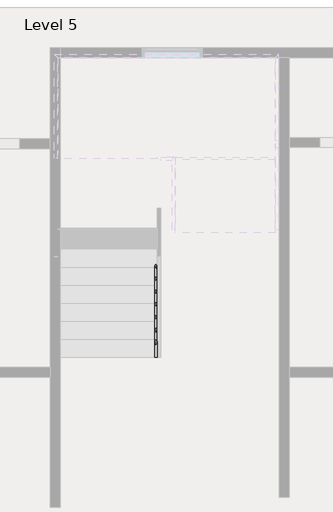
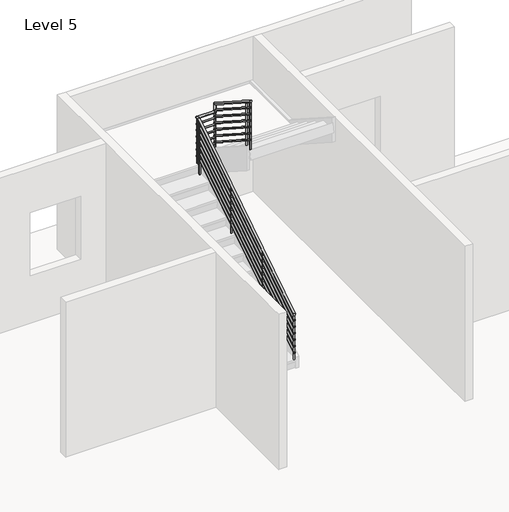
# One storey, part 6 of 7: 1 railing.
"""IFC4 building model written with IfcOpenShell, lengths in millimetres."""

from ifc_helpers import new_model, si_unit, point, frame, frame_2d, origin, place, context, project, spatial, circle_curve, ellipse_curve, trimmed, segment, composite_curve, outline, extrude, element, save
from ifc_brep_helpers import plane_surface, cylinder_surface, advanced_brep

model = new_model("IFC4")

# Units and contexts
model_context = context("Model", 3, world=origin())
ifc_project = project(units=[si_unit("LENGTHUNIT", "METRE", prefix="MILLI")], contexts=[model_context])

# Site, building, storey
site = spatial("IfcSite", under=ifc_project)
building = spatial("IfcBuilding", under=site)
storey = spatial("IfcBuildingStorey", under=building, Name="Level 5", Elevation=12500.0)

# Railing
placement = place(None, origin())
element("IfcRailing", 1, ObjectType="900mm Pipe", at=placement, inside=storey, context=model_context, shape_type="SolidModel", body=[
    advanced_brep(
    [(-504.8393676, 4284.7509075, 13552.7068065), (-544.8393676, 4284.7509075, 13552.7068065), (-504.8393676, 7315.616134, 15497.6470588), (-544.8393676, 7315.616134, 15497.6470588), (-504.8393676, 7337.8781803, 15497.6470588), (-544.8393676, 7377.8781803, 15497.6470588), (-201.3120949, 7337.8781803, 15497.6470588), (-201.3120949, 7377.8781803, 15497.6470588)],
    [
        (0, 1, ellipse_curve(frame((-524.8393676, 4284.7509075, 13552.7068065), z_axis=(0.0, -1.0, 0.0), x_axis=(0.0, 0.0, -1.0)), 23.7637817, 20.0)),
        (1, 0, ellipse_curve(frame((-524.8393676, 4284.7509075, 13552.7068065), z_axis=(0.0, -1.0, 0.0), x_axis=(0.0, 0.0, -1.0)), 23.7637817, 20.0)),
        (0, 2),
        (2, 3, ellipse_curve(frame((-524.8393676, 7315.616134, 15497.6470588), z_axis=(0.0, -0.9595876426002529, -0.28140994326585084), x_axis=(0.0, 0.2814099432658509, -0.959587642600253)), 20.8422859, 20.0)),
        (3, 1),
        (3, 2, ellipse_curve(frame((-524.8393676, 7315.616134, 15497.6470588), z_axis=(0.0, -0.9595876426002529, -0.28140994326585084), x_axis=(0.0, 0.2814099432658509, -0.959587642600253)), 20.8422859, 20.0)),
        (2, 4),
        (4, 5, ellipse_curve(frame((-524.8393676, 7357.8781803, 15497.6470588), z_axis=(-0.7071067811865475, -0.7071067811865475, 0.0), x_axis=(0.7071067811865474, -0.7071067811865476, 0.0)), 28.2842712, 20.0)),
        (5, 3),
        (5, 4, ellipse_curve(frame((-524.8393676, 7357.8781803, 15497.6470588), z_axis=(-0.7071067811865475, -0.7071067811865475, 0.0), x_axis=(0.7071067811865474, -0.7071067811865476, 0.0)), 28.2842712, 20.0)),
        (6, 7, ellipse_curve(frame((-201.3120949, 7357.8781803, 15497.6470588), z_axis=(0.7071067811865476, 0.0, 0.7071067811865476), x_axis=(-0.7071067811865474, 0.0, 0.7071067811865476)), 28.2842712, 20.0)),
        (7, 6, ellipse_curve(frame((-201.3120949, 7357.8781803, 15497.6470588), z_axis=(0.7071067811865476, 0.0, 0.7071067811865476), x_axis=(-0.7071067811865474, 0.0, 0.7071067811865476)), 28.2842712, 20.0)),
        (4, 6),
        (7, 5),
    ],
    [
        plane_surface(frame((-524.8393676, 4284.7509075, 13576.4705882), z_axis=(0.0, -1.0, 0.0), x_axis=(0.0, 0.0, 1.0))),
        cylinder_surface(frame((-524.8393676, 4295.5524077, 13559.6382505), z_axis=(0.0, -0.8416168876622212, -0.5400750081254975), x_axis=(-1.0, 0.0, 0.0)), 20.0),
        cylinder_surface(frame((-524.8393676, 7309.7509075, 15497.6470588), z_axis=(0.0, -1.0, 0.0), x_axis=(-1.0, 0.0, 0.0)), 20.0),
        plane_surface(frame((-221.3120949, 7357.8781803, 15517.6470588), z_axis=(0.7071067811865476, 0.0, 0.7071067811865476), x_axis=(0.7071067811865476, 0.0, -0.7071067811865476))),
        cylinder_surface(frame((-524.8393676, 7357.8781803, 15497.6470588), z_axis=(-1.0, 0.0, 0.0), x_axis=(0.0, 1.0, 0.0)), 20.0),
    ],
    [
        (0, [[1, 2]]),
        (1, [[-1, 3, 4, 5]]),
        (1, [[-2, -5, 6, -3]]),
        (2, [[-4, 7, 8, 9]]),
        (2, [[-6, -9, 10, -7]]),
        (3, [[11, 12]]),
        (4, [[-8, 13, -12, 14]]),
        (4, [[-10, -14, -11, -13]]),
    ],
),
    advanced_brep(
    [(-201.3120949, 7337.8781803, 15497.6470588), (-201.3120949, 7377.8781803, 15497.6470588), (-201.3120949, 7337.8781803, 15643.124843), (-201.3120949, 7377.8781803, 15664.9839572)],
    [
        (0, 1, ellipse_curve(frame((-201.3120949, 7357.8781803, 15497.6470588), z_axis=(-0.7071067811865476, 0.0, -0.7071067811865476), x_axis=(0.7071067811865476, 0.0, -0.7071067811865474)), 28.2842712, 20.0)),
        (1, 0, ellipse_curve(frame((-201.3120949, 7357.8781803, 15497.6470588), z_axis=(-0.7071067811865476, 0.0, -0.7071067811865476), x_axis=(0.7071067811865476, 0.0, -0.7071067811865474)), 28.2842712, 20.0)),
        (2, 3, ellipse_curve(frame((-201.3120949, 7357.8781803, 15654.0544001), z_axis=(0.0, -0.47954405004884676, 0.877517808402057), x_axis=(0.0, -0.8775178084020571, -0.47954405004884676)), 22.7915602, 20.0)),
        (3, 2, ellipse_curve(frame((-201.3120949, 7357.8781803, 15654.0544001), z_axis=(0.0, -0.47954405004884676, 0.877517808402057), x_axis=(0.0, -0.8775178084020571, -0.47954405004884676)), 22.7915602, 20.0)),
        (0, 2),
        (3, 1),
    ],
    [
        plane_surface(frame((-201.3120949, 7357.8781803, 15497.6470588), z_axis=(-0.7071067811865476, 0.0, -0.7071067811865476), x_axis=(0.7071067811865476, 0.0, -0.7071067811865476))),
        plane_surface(frame((-201.3120949, 7357.8781803, 15654.0544001), z_axis=(0.0, -0.47954405004884676, 0.877517808402057), x_axis=(1.0, 0.0, 0.0))),
        cylinder_surface(frame((-201.3120949, 7357.8781803, 15497.6470588), z_axis=(0.0, 0.0, -1.0), x_axis=(0.0, 1.0, 0.0)), 20.0),
    ],
    [
        (0, [[1, 2]]),
        (1, [[3, 4]]),
        (2, [[-1, 5, -4, 6]]),
        (2, [[-2, -6, -3, -5]]),
    ],
),
    advanced_brep(
    [(-221.3120949, 7357.8781803, 15654.0544001), (-181.3120949, 7357.8781803, 15654.0544001), (-221.3120949, 6232.4781803, 16376.2362183), (-181.3120949, 6232.4781803, 16376.2362183)],
    [
        (0, 1, ellipse_curve(frame((-201.3120949, 7357.8781803, 15654.0544001), z_axis=(0.0, 0.47954405004884676, -0.877517808402057), x_axis=(0.0, 0.8775178084020568, 0.47954405004884676)), 22.7915602, 20.0)),
        (1, 0, ellipse_curve(frame((-201.3120949, 7357.8781803, 15654.0544001), z_axis=(0.0, 0.47954405004884676, -0.877517808402057), x_axis=(0.0, 0.8775178084020568, 0.47954405004884676)), 22.7915602, 20.0)),
        (2, 3, ellipse_curve(frame((-201.3120949, 6232.4781803, 16376.2362183), z_axis=(0.0, -1.0, 0.0), x_axis=(0.0, 0.0, -1.0)), 23.7637817, 20.0)),
        (3, 2, ellipse_curve(frame((-201.3120949, 6232.4781803, 16376.2362183), z_axis=(0.0, -1.0, 0.0), x_axis=(0.0, 0.0, -1.0)), 23.7637817, 20.0)),
        (0, 2),
        (3, 1),
    ],
    [
        plane_surface(frame((-201.3120949, 7377.8781803, 15664.9839572), z_axis=(0.0, 0.47954405004884676, -0.877517808402057), x_axis=(1.0, 0.0, 0.0))),
        plane_surface(frame((-201.3120949, 6232.4781803, 16400.0), z_axis=(0.0, -1.0, 0.0), x_axis=(0.0, 0.0, -1.0))),
        cylinder_surface(frame((-201.3120949, 7367.0766801, 15648.1516195), z_axis=(0.0, 0.8416168876622208, -0.5400750081254984), x_axis=(1.0, 0.0, 0.0)), 20.0),
    ],
    [
        (0, [[1, 2]]),
        (1, [[3, 4]]),
        (2, [[-1, 5, -4, 6]]),
        (2, [[-2, -6, -3, -5]]),
    ],
),
    advanced_brep(
    [(-539.8393676, 4284.7509075, 13433.647752), (-509.8393676, 4284.7509075, 13433.647752), (-539.8393676, 7309.7509075, 15374.8242225), (-509.8393676, 7309.7509075, 15374.8242225)],
    [
        (0, 1, ellipse_curve(frame((-524.8393676, 4284.7509075, 13433.647752), z_axis=(0.0, -1.0, 0.0), x_axis=(0.0, 0.0, -1.0)), 17.8228363, 15.0)),
        (1, 0, ellipse_curve(frame((-524.8393676, 4284.7509075, 13433.647752), z_axis=(0.0, -1.0, 0.0), x_axis=(0.0, 0.0, -1.0)), 17.8228363, 15.0)),
        (2, 3, ellipse_curve(frame((-524.8393676, 7309.7509075, 15374.8242225), z_axis=(0.0, 1.0, 0.0), x_axis=(0.0, 0.0, -1.0)), 17.8228363, 15.0)),
        (3, 2, ellipse_curve(frame((-524.8393676, 7309.7509075, 15374.8242225), z_axis=(0.0, 1.0, 0.0), x_axis=(0.0, 0.0, -1.0)), 17.8228363, 15.0)),
        (0, 2),
        (3, 1),
    ],
    [
        plane_surface(frame((-524.8393676, 4284.7509075, 13451.4705882), z_axis=(0.0, -1.0, 0.0), x_axis=(0.0, 0.0, 1.0))),
        plane_surface(frame((-524.8393676, 7309.7509075, 15392.6470588), z_axis=(0.0, 1.0, 0.0), x_axis=(0.0, 0.0, 1.0))),
        cylinder_surface(frame((-524.8393676, 4292.8520327, 13438.8463349), z_axis=(0.0, -0.8416168876622212, -0.5400750081254975), x_axis=(1.0, 0.0, 0.0)), 15.0),
    ],
    [
        (0, [[1, 2]]),
        (1, [[3, 4]]),
        (2, [[-1, 5, -4, 6]]),
        (2, [[-2, -6, -3, -5]]),
    ],
),
    advanced_brep(
    [(-539.8393676, 7309.7509075, 15377.6470588), (-509.8393676, 7309.7509075, 15377.6470588), (-539.8393676, 7342.8781803, 15377.6470588), (-509.8393676, 7342.8781803, 15377.6470588)],
    [
        (0, 1, circle_curve(frame((-524.8393676, 7309.7509075, 15377.6470588), z_axis=(0.0, -1.0, 0.0), x_axis=(1.0, 0.0, 0.0)), 15.0)),
        (1, 0, circle_curve(frame((-524.8393676, 7309.7509075, 15377.6470588), z_axis=(0.0, -1.0, 0.0), x_axis=(1.0, 0.0, 0.0)), 15.0)),
        (2, 3, circle_curve(frame((-524.8393676, 7342.8781803, 15377.6470588), z_axis=(0.0, 1.0, 0.0), x_axis=(1.0, 0.0, 0.0)), 15.0)),
        (3, 2, circle_curve(frame((-524.8393676, 7342.8781803, 15377.6470588), z_axis=(0.0, 1.0, 0.0), x_axis=(1.0, 0.0, 0.0)), 15.0)),
        (0, 2),
        (3, 1),
    ],
    [
        plane_surface(frame((-524.8393676, 7309.7509075, 15392.6470588), z_axis=(0.0, -1.0, 0.0), x_axis=(0.0, 0.0, 1.0))),
        plane_surface(frame((-524.8393676, 7342.8781803, 15392.6470588), z_axis=(0.0, 1.0, 0.0), x_axis=(0.0, 0.0, 1.0))),
        cylinder_surface(frame((-524.8393676, 7309.7509075, 15377.6470588), z_axis=(0.0, -1.0, 0.0), x_axis=(1.0, 0.0, 0.0)), 15.0),
    ],
    [
        (0, [[1, 2]]),
        (1, [[3, 4]]),
        (2, [[-1, 5, -4, 6]]),
        (2, [[-2, -6, -3, -5]]),
    ],
),
    advanced_brep(
    [(-539.8393676, 7372.8781803, 15377.6470588), (-539.8393676, 7342.8781803, 15377.6470588), (-216.3120949, 7372.8781803, 15377.6470588), (-216.3120949, 7342.8781803, 15377.6470588)],
    [
        (0, 1, circle_curve(frame((-539.8393676, 7357.8781803, 15377.6470588), z_axis=(-1.0, 0.0, 0.0), x_axis=(0.0, -1.0, 0.0)), 15.0)),
        (1, 0, circle_curve(frame((-539.8393676, 7357.8781803, 15377.6470588), z_axis=(-1.0, 0.0, 0.0), x_axis=(0.0, -1.0, 0.0)), 15.0)),
        (2, 3, circle_curve(frame((-216.3120949, 7357.8781803, 15377.6470588), z_axis=(1.0, 0.0, 0.0), x_axis=(0.0, -1.0, 0.0)), 15.0)),
        (3, 2, circle_curve(frame((-216.3120949, 7357.8781803, 15377.6470588), z_axis=(1.0, 0.0, 0.0), x_axis=(0.0, -1.0, 0.0)), 15.0)),
        (0, 2),
        (3, 1),
    ],
    [
        plane_surface(frame((-539.8393676, 7357.8781803, 15392.6470588), z_axis=(-1.0, 0.0, 0.0), x_axis=(0.0, 1.0, 0.0))),
        plane_surface(frame((-216.3120949, 7357.8781803, 15392.6470588), z_axis=(1.0, 0.0, 0.0), x_axis=(0.0, 1.0, 0.0))),
        cylinder_surface(frame((-539.8393676, 7357.8781803, 15377.6470588), z_axis=(-1.0, 0.0, 0.0), x_axis=(0.0, -1.0, 0.0)), 15.0),
    ],
    [
        (0, [[1, 2]]),
        (1, [[3, 4]]),
        (2, [[-1, 5, -4, 6]]),
        (2, [[-2, -6, -3, -5]]),
    ],
),
    advanced_brep(
    [(-186.3120949, 7372.8781803, 15525.3696771), (-216.3120949, 7372.8781803, 15525.3696771), (-186.3120949, 6232.4781803, 16257.1771637), (-216.3120949, 6232.4781803, 16257.1771637)],
    [
        (0, 1, ellipse_curve(frame((-201.3120949, 7372.8781803, 15525.3696771), z_axis=(0.0, 1.0, 0.0), x_axis=(0.0, 0.0, -1.0)), 17.8228363, 15.0)),
        (1, 0, ellipse_curve(frame((-201.3120949, 7372.8781803, 15525.3696771), z_axis=(0.0, 1.0, 0.0), x_axis=(0.0, 0.0, -1.0)), 17.8228363, 15.0)),
        (2, 3, ellipse_curve(frame((-201.3120949, 6232.4781803, 16257.1771637), z_axis=(0.0, -1.0, 0.0), x_axis=(0.0, 0.0, -1.0)), 17.8228363, 15.0)),
        (3, 2, ellipse_curve(frame((-201.3120949, 6232.4781803, 16257.1771637), z_axis=(0.0, -1.0, 0.0), x_axis=(0.0, 0.0, -1.0)), 17.8228363, 15.0)),
        (0, 2),
        (3, 1),
    ],
    [
        plane_surface(frame((-201.3120949, 7372.8781803, 15543.1925134), z_axis=(0.0, 1.0, 0.0), x_axis=(0.0, 0.0, -1.0))),
        plane_surface(frame((-201.3120949, 6232.4781803, 16275.0), z_axis=(0.0, -1.0, 0.0), x_axis=(0.0, 0.0, -1.0))),
        cylinder_surface(frame((-201.3120949, 7364.7770552, 15530.5682601), z_axis=(0.0, 0.8416168876622208, -0.5400750081254984), x_axis=(-1.0, 0.0, 0.0)), 15.0),
    ],
    [
        (0, [[1, 2]]),
        (1, [[3, 4]]),
        (2, [[-1, 5, -4, 6]]),
        (2, [[-2, -6, -3, -5]]),
    ],
),
    advanced_brep(
    [(-539.8393676, 4284.7509075, 13308.647752), (-509.8393676, 4284.7509075, 13308.647752), (-539.8393676, 7309.7509075, 15249.8242225), (-509.8393676, 7309.7509075, 15249.8242225)],
    [
        (0, 1, ellipse_curve(frame((-524.8393676, 4284.7509075, 13308.647752), z_axis=(0.0, -1.0, 0.0), x_axis=(0.0, 0.0, -1.0)), 17.8228363, 15.0)),
        (1, 0, ellipse_curve(frame((-524.8393676, 4284.7509075, 13308.647752), z_axis=(0.0, -1.0, 0.0), x_axis=(0.0, 0.0, -1.0)), 17.8228363, 15.0)),
        (2, 3, ellipse_curve(frame((-524.8393676, 7309.7509075, 15249.8242225), z_axis=(0.0, 1.0, 0.0), x_axis=(0.0, 0.0, -1.0)), 17.8228363, 15.0)),
        (3, 2, ellipse_curve(frame((-524.8393676, 7309.7509075, 15249.8242225), z_axis=(0.0, 1.0, 0.0), x_axis=(0.0, 0.0, -1.0)), 17.8228363, 15.0)),
        (0, 2),
        (3, 1),
    ],
    [
        plane_surface(frame((-524.8393676, 4284.7509075, 13326.4705882), z_axis=(0.0, -1.0, 0.0), x_axis=(0.0, 0.0, 1.0))),
        plane_surface(frame((-524.8393676, 7309.7509075, 15267.6470588), z_axis=(0.0, 1.0, 0.0), x_axis=(0.0, 0.0, 1.0))),
        cylinder_surface(frame((-524.8393676, 4292.8520327, 13313.8463349), z_axis=(0.0, -0.8416168876622212, -0.5400750081254975), x_axis=(1.0, 0.0, 0.0)), 15.0),
    ],
    [
        (0, [[1, 2]]),
        (1, [[3, 4]]),
        (2, [[-1, 5, -4, 6]]),
        (2, [[-2, -6, -3, -5]]),
    ],
),
    advanced_brep(
    [(-539.8393676, 7309.7509075, 15252.6470588), (-509.8393676, 7309.7509075, 15252.6470588), (-539.8393676, 7342.8781803, 15252.6470588), (-509.8393676, 7342.8781803, 15252.6470588)],
    [
        (0, 1, circle_curve(frame((-524.8393676, 7309.7509075, 15252.6470588), z_axis=(0.0, -1.0, 0.0), x_axis=(1.0, 0.0, 0.0)), 15.0)),
        (1, 0, circle_curve(frame((-524.8393676, 7309.7509075, 15252.6470588), z_axis=(0.0, -1.0, 0.0), x_axis=(1.0, 0.0, 0.0)), 15.0)),
        (2, 3, circle_curve(frame((-524.8393676, 7342.8781803, 15252.6470588), z_axis=(0.0, 1.0, 0.0), x_axis=(1.0, 0.0, 0.0)), 15.0)),
        (3, 2, circle_curve(frame((-524.8393676, 7342.8781803, 15252.6470588), z_axis=(0.0, 1.0, 0.0), x_axis=(1.0, 0.0, 0.0)), 15.0)),
        (0, 2),
        (3, 1),
    ],
    [
        plane_surface(frame((-524.8393676, 7309.7509075, 15267.6470588), z_axis=(0.0, -1.0, 0.0), x_axis=(0.0, 0.0, 1.0))),
        plane_surface(frame((-524.8393676, 7342.8781803, 15267.6470588), z_axis=(0.0, 1.0, 0.0), x_axis=(0.0, 0.0, 1.0))),
        cylinder_surface(frame((-524.8393676, 7309.7509075, 15252.6470588), z_axis=(0.0, -1.0, 0.0), x_axis=(1.0, 0.0, 0.0)), 15.0),
    ],
    [
        (0, [[1, 2]]),
        (1, [[3, 4]]),
        (2, [[-1, 5, -4, 6]]),
        (2, [[-2, -6, -3, -5]]),
    ],
),
    advanced_brep(
    [(-539.8393676, 7372.8781803, 15252.6470588), (-539.8393676, 7342.8781803, 15252.6470588), (-216.3120949, 7372.8781803, 15252.6470588), (-216.3120949, 7342.8781803, 15252.6470588)],
    [
        (0, 1, circle_curve(frame((-539.8393676, 7357.8781803, 15252.6470588), z_axis=(-1.0, 0.0, 0.0), x_axis=(0.0, -1.0, 0.0)), 15.0)),
        (1, 0, circle_curve(frame((-539.8393676, 7357.8781803, 15252.6470588), z_axis=(-1.0, 0.0, 0.0), x_axis=(0.0, -1.0, 0.0)), 15.0)),
        (2, 3, circle_curve(frame((-216.3120949, 7357.8781803, 15252.6470588), z_axis=(1.0, 0.0, 0.0), x_axis=(0.0, -1.0, 0.0)), 15.0)),
        (3, 2, circle_curve(frame((-216.3120949, 7357.8781803, 15252.6470588), z_axis=(1.0, 0.0, 0.0), x_axis=(0.0, -1.0, 0.0)), 15.0)),
        (0, 2),
        (3, 1),
    ],
    [
        plane_surface(frame((-539.8393676, 7357.8781803, 15267.6470588), z_axis=(-1.0, 0.0, 0.0), x_axis=(0.0, 1.0, 0.0))),
        plane_surface(frame((-216.3120949, 7357.8781803, 15267.6470588), z_axis=(1.0, 0.0, 0.0), x_axis=(0.0, 1.0, 0.0))),
        cylinder_surface(frame((-539.8393676, 7357.8781803, 15252.6470588), z_axis=(-1.0, 0.0, 0.0), x_axis=(0.0, -1.0, 0.0)), 15.0),
    ],
    [
        (0, [[1, 2]]),
        (1, [[3, 4]]),
        (2, [[-1, 5, -4, 6]]),
        (2, [[-2, -6, -3, -5]]),
    ],
),
    advanced_brep(
    [(-186.3120949, 7372.8781803, 15400.3696771), (-216.3120949, 7372.8781803, 15400.3696771), (-186.3120949, 6232.4781803, 16132.1771637), (-216.3120949, 6232.4781803, 16132.1771637)],
    [
        (0, 1, ellipse_curve(frame((-201.3120949, 7372.8781803, 15400.3696771), z_axis=(0.0, 1.0, 0.0), x_axis=(0.0, 0.0, -1.0)), 17.8228363, 15.0)),
        (1, 0, ellipse_curve(frame((-201.3120949, 7372.8781803, 15400.3696771), z_axis=(0.0, 1.0, 0.0), x_axis=(0.0, 0.0, -1.0)), 17.8228363, 15.0)),
        (2, 3, ellipse_curve(frame((-201.3120949, 6232.4781803, 16132.1771637), z_axis=(0.0, -1.0, 0.0), x_axis=(0.0, 0.0, -1.0)), 17.8228363, 15.0)),
        (3, 2, ellipse_curve(frame((-201.3120949, 6232.4781803, 16132.1771637), z_axis=(0.0, -1.0, 0.0), x_axis=(0.0, 0.0, -1.0)), 17.8228363, 15.0)),
        (0, 2),
        (3, 1),
    ],
    [
        plane_surface(frame((-201.3120949, 7372.8781803, 15418.1925134), z_axis=(0.0, 1.0, 0.0), x_axis=(0.0, 0.0, -1.0))),
        plane_surface(frame((-201.3120949, 6232.4781803, 16150.0), z_axis=(0.0, -1.0, 0.0), x_axis=(0.0, 0.0, -1.0))),
        cylinder_surface(frame((-201.3120949, 7364.7770552, 15405.5682601), z_axis=(0.0, 0.8416168876622208, -0.5400750081254984), x_axis=(-1.0, 0.0, 0.0)), 15.0),
    ],
    [
        (0, [[1, 2]]),
        (1, [[3, 4]]),
        (2, [[-1, 5, -4, 6]]),
        (2, [[-2, -6, -3, -5]]),
    ],
),
    advanced_brep(
    [(-539.8393676, 4284.7509075, 13183.647752), (-509.8393676, 4284.7509075, 13183.647752), (-539.8393676, 7309.7509075, 15124.8242225), (-509.8393676, 7309.7509075, 15124.8242225)],
    [
        (0, 1, ellipse_curve(frame((-524.8393676, 4284.7509075, 13183.647752), z_axis=(0.0, -1.0, 0.0), x_axis=(0.0, 0.0, -1.0)), 17.8228363, 15.0)),
        (1, 0, ellipse_curve(frame((-524.8393676, 4284.7509075, 13183.647752), z_axis=(0.0, -1.0, 0.0), x_axis=(0.0, 0.0, -1.0)), 17.8228363, 15.0)),
        (2, 3, ellipse_curve(frame((-524.8393676, 7309.7509075, 15124.8242225), z_axis=(0.0, 1.0, 0.0), x_axis=(0.0, 0.0, -1.0)), 17.8228363, 15.0)),
        (3, 2, ellipse_curve(frame((-524.8393676, 7309.7509075, 15124.8242225), z_axis=(0.0, 1.0, 0.0), x_axis=(0.0, 0.0, -1.0)), 17.8228363, 15.0)),
        (0, 2),
        (3, 1),
    ],
    [
        plane_surface(frame((-524.8393676, 4284.7509075, 13201.4705882), z_axis=(0.0, -1.0, 0.0), x_axis=(0.0, 0.0, 1.0))),
        plane_surface(frame((-524.8393676, 7309.7509075, 15142.6470588), z_axis=(0.0, 1.0, 0.0), x_axis=(0.0, 0.0, 1.0))),
        cylinder_surface(frame((-524.8393676, 4292.8520327, 13188.8463349), z_axis=(0.0, -0.8416168876622212, -0.5400750081254975), x_axis=(1.0, 0.0, 0.0)), 15.0),
    ],
    [
        (0, [[1, 2]]),
        (1, [[3, 4]]),
        (2, [[-1, 5, -4, 6]]),
        (2, [[-2, -6, -3, -5]]),
    ],
),
    advanced_brep(
    [(-539.8393676, 7309.7509075, 15127.6470588), (-509.8393676, 7309.7509075, 15127.6470588), (-539.8393676, 7342.8781803, 15127.6470588), (-509.8393676, 7342.8781803, 15127.6470588)],
    [
        (0, 1, circle_curve(frame((-524.8393676, 7309.7509075, 15127.6470588), z_axis=(0.0, -1.0, 0.0), x_axis=(1.0, 0.0, 0.0)), 15.0)),
        (1, 0, circle_curve(frame((-524.8393676, 7309.7509075, 15127.6470588), z_axis=(0.0, -1.0, 0.0), x_axis=(1.0, 0.0, 0.0)), 15.0)),
        (2, 3, circle_curve(frame((-524.8393676, 7342.8781803, 15127.6470588), z_axis=(0.0, 1.0, 0.0), x_axis=(1.0, 0.0, 0.0)), 15.0)),
        (3, 2, circle_curve(frame((-524.8393676, 7342.8781803, 15127.6470588), z_axis=(0.0, 1.0, 0.0), x_axis=(1.0, 0.0, 0.0)), 15.0)),
        (0, 2),
        (3, 1),
    ],
    [
        plane_surface(frame((-524.8393676, 7309.7509075, 15142.6470588), z_axis=(0.0, -1.0, 0.0), x_axis=(0.0, 0.0, 1.0))),
        plane_surface(frame((-524.8393676, 7342.8781803, 15142.6470588), z_axis=(0.0, 1.0, 0.0), x_axis=(0.0, 0.0, 1.0))),
        cylinder_surface(frame((-524.8393676, 7309.7509075, 15127.6470588), z_axis=(0.0, -1.0, 0.0), x_axis=(1.0, 0.0, 0.0)), 15.0),
    ],
    [
        (0, [[1, 2]]),
        (1, [[3, 4]]),
        (2, [[-1, 5, -4, 6]]),
        (2, [[-2, -6, -3, -5]]),
    ],
),
    advanced_brep(
    [(-539.8393676, 7372.8781803, 15127.6470588), (-539.8393676, 7342.8781803, 15127.6470588), (-216.3120949, 7372.8781803, 15127.6470588), (-216.3120949, 7342.8781803, 15127.6470588)],
    [
        (0, 1, circle_curve(frame((-539.8393676, 7357.8781803, 15127.6470588), z_axis=(-1.0, 0.0, 0.0), x_axis=(0.0, -1.0, 0.0)), 15.0)),
        (1, 0, circle_curve(frame((-539.8393676, 7357.8781803, 15127.6470588), z_axis=(-1.0, 0.0, 0.0), x_axis=(0.0, -1.0, 0.0)), 15.0)),
        (2, 3, circle_curve(frame((-216.3120949, 7357.8781803, 15127.6470588), z_axis=(1.0, 0.0, 0.0), x_axis=(0.0, -1.0, 0.0)), 15.0)),
        (3, 2, circle_curve(frame((-216.3120949, 7357.8781803, 15127.6470588), z_axis=(1.0, 0.0, 0.0), x_axis=(0.0, -1.0, 0.0)), 15.0)),
        (0, 2),
        (3, 1),
    ],
    [
        plane_surface(frame((-539.8393676, 7357.8781803, 15142.6470588), z_axis=(-1.0, 0.0, 0.0), x_axis=(0.0, 1.0, 0.0))),
        plane_surface(frame((-216.3120949, 7357.8781803, 15142.6470588), z_axis=(1.0, 0.0, 0.0), x_axis=(0.0, 1.0, 0.0))),
        cylinder_surface(frame((-539.8393676, 7357.8781803, 15127.6470588), z_axis=(-1.0, 0.0, 0.0), x_axis=(0.0, -1.0, 0.0)), 15.0),
    ],
    [
        (0, [[1, 2]]),
        (1, [[3, 4]]),
        (2, [[-1, 5, -4, 6]]),
        (2, [[-2, -6, -3, -5]]),
    ],
),
    advanced_brep(
    [(-186.3120949, 7372.8781803, 15275.3696771), (-216.3120949, 7372.8781803, 15275.3696771), (-186.3120949, 6232.4781803, 16007.1771637), (-216.3120949, 6232.4781803, 16007.1771637)],
    [
        (0, 1, ellipse_curve(frame((-201.3120949, 7372.8781803, 15275.3696771), z_axis=(0.0, 1.0, 0.0), x_axis=(0.0, 0.0, -1.0)), 17.8228363, 15.0)),
        (1, 0, ellipse_curve(frame((-201.3120949, 7372.8781803, 15275.3696771), z_axis=(0.0, 1.0, 0.0), x_axis=(0.0, 0.0, -1.0)), 17.8228363, 15.0)),
        (2, 3, ellipse_curve(frame((-201.3120949, 6232.4781803, 16007.1771637), z_axis=(0.0, -1.0, 0.0), x_axis=(0.0, 0.0, -1.0)), 17.8228363, 15.0)),
        (3, 2, ellipse_curve(frame((-201.3120949, 6232.4781803, 16007.1771637), z_axis=(0.0, -1.0, 0.0), x_axis=(0.0, 0.0, -1.0)), 17.8228363, 15.0)),
        (0, 2),
        (3, 1),
    ],
    [
        plane_surface(frame((-201.3120949, 7372.8781803, 15293.1925134), z_axis=(0.0, 1.0, 0.0), x_axis=(0.0, 0.0, -1.0))),
        plane_surface(frame((-201.3120949, 6232.4781803, 16025.0), z_axis=(0.0, -1.0, 0.0), x_axis=(0.0, 0.0, -1.0))),
        cylinder_surface(frame((-201.3120949, 7364.7770552, 15280.5682601), z_axis=(0.0, 0.8416168876622208, -0.5400750081254984), x_axis=(-1.0, 0.0, 0.0)), 15.0),
    ],
    [
        (0, [[1, 2]]),
        (1, [[3, 4]]),
        (2, [[-1, 5, -4, 6]]),
        (2, [[-2, -6, -3, -5]]),
    ],
),
    advanced_brep(
    [(-539.8393676, 4284.7509075, 13058.647752), (-509.8393676, 4284.7509075, 13058.647752), (-539.8393676, 7309.7509075, 14999.8242225), (-509.8393676, 7309.7509075, 14999.8242225)],
    [
        (0, 1, ellipse_curve(frame((-524.8393676, 4284.7509075, 13058.647752), z_axis=(0.0, -1.0, 0.0), x_axis=(0.0, 0.0, -1.0)), 17.8228363, 15.0)),
        (1, 0, ellipse_curve(frame((-524.8393676, 4284.7509075, 13058.647752), z_axis=(0.0, -1.0, 0.0), x_axis=(0.0, 0.0, -1.0)), 17.8228363, 15.0)),
        (2, 3, ellipse_curve(frame((-524.8393676, 7309.7509075, 14999.8242225), z_axis=(0.0, 1.0, 0.0), x_axis=(0.0, 0.0, -1.0)), 17.8228363, 15.0)),
        (3, 2, ellipse_curve(frame((-524.8393676, 7309.7509075, 14999.8242225), z_axis=(0.0, 1.0, 0.0), x_axis=(0.0, 0.0, -1.0)), 17.8228363, 15.0)),
        (0, 2),
        (3, 1),
    ],
    [
        plane_surface(frame((-524.8393676, 4284.7509075, 13076.4705882), z_axis=(0.0, -1.0, 0.0), x_axis=(0.0, 0.0, 1.0))),
        plane_surface(frame((-524.8393676, 7309.7509075, 15017.6470588), z_axis=(0.0, 1.0, 0.0), x_axis=(0.0, 0.0, 1.0))),
        cylinder_surface(frame((-524.8393676, 4292.8520327, 13063.8463349), z_axis=(0.0, -0.8416168876622212, -0.5400750081254975), x_axis=(1.0, 0.0, 0.0)), 15.0),
    ],
    [
        (0, [[1, 2]]),
        (1, [[3, 4]]),
        (2, [[-1, 5, -4, 6]]),
        (2, [[-2, -6, -3, -5]]),
    ],
),
    advanced_brep(
    [(-539.8393676, 7309.7509075, 15002.6470588), (-509.8393676, 7309.7509075, 15002.6470588), (-539.8393676, 7342.8781803, 15002.6470588), (-509.8393676, 7342.8781803, 15002.6470588)],
    [
        (0, 1, circle_curve(frame((-524.8393676, 7309.7509075, 15002.6470588), z_axis=(0.0, -1.0, 0.0), x_axis=(1.0, 0.0, 0.0)), 15.0)),
        (1, 0, circle_curve(frame((-524.8393676, 7309.7509075, 15002.6470588), z_axis=(0.0, -1.0, 0.0), x_axis=(1.0, 0.0, 0.0)), 15.0)),
        (2, 3, circle_curve(frame((-524.8393676, 7342.8781803, 15002.6470588), z_axis=(0.0, 1.0, 0.0), x_axis=(1.0, 0.0, 0.0)), 15.0)),
        (3, 2, circle_curve(frame((-524.8393676, 7342.8781803, 15002.6470588), z_axis=(0.0, 1.0, 0.0), x_axis=(1.0, 0.0, 0.0)), 15.0)),
        (0, 2),
        (3, 1),
    ],
    [
        plane_surface(frame((-524.8393676, 7309.7509075, 15017.6470588), z_axis=(0.0, -1.0, 0.0), x_axis=(0.0, 0.0, 1.0))),
        plane_surface(frame((-524.8393676, 7342.8781803, 15017.6470588), z_axis=(0.0, 1.0, 0.0), x_axis=(0.0, 0.0, 1.0))),
        cylinder_surface(frame((-524.8393676, 7309.7509075, 15002.6470588), z_axis=(0.0, -1.0, 0.0), x_axis=(1.0, 0.0, 0.0)), 15.0),
    ],
    [
        (0, [[1, 2]]),
        (1, [[3, 4]]),
        (2, [[-1, 5, -4, 6]]),
        (2, [[-2, -6, -3, -5]]),
    ],
),
    advanced_brep(
    [(-539.8393676, 7372.8781803, 15002.6470588), (-539.8393676, 7342.8781803, 15002.6470588), (-216.3120949, 7372.8781803, 15002.6470588), (-216.3120949, 7342.8781803, 15002.6470588)],
    [
        (0, 1, circle_curve(frame((-539.8393676, 7357.8781803, 15002.6470588), z_axis=(-1.0, 0.0, 0.0), x_axis=(0.0, -1.0, 0.0)), 15.0)),
        (1, 0, circle_curve(frame((-539.8393676, 7357.8781803, 15002.6470588), z_axis=(-1.0, 0.0, 0.0), x_axis=(0.0, -1.0, 0.0)), 15.0)),
        (2, 3, circle_curve(frame((-216.3120949, 7357.8781803, 15002.6470588), z_axis=(1.0, 0.0, 0.0), x_axis=(0.0, -1.0, 0.0)), 15.0)),
        (3, 2, circle_curve(frame((-216.3120949, 7357.8781803, 15002.6470588), z_axis=(1.0, 0.0, 0.0), x_axis=(0.0, -1.0, 0.0)), 15.0)),
        (0, 2),
        (3, 1),
    ],
    [
        plane_surface(frame((-539.8393676, 7357.8781803, 15017.6470588), z_axis=(-1.0, 0.0, 0.0), x_axis=(0.0, 1.0, 0.0))),
        plane_surface(frame((-216.3120949, 7357.8781803, 15017.6470588), z_axis=(1.0, 0.0, 0.0), x_axis=(0.0, 1.0, 0.0))),
        cylinder_surface(frame((-539.8393676, 7357.8781803, 15002.6470588), z_axis=(-1.0, 0.0, 0.0), x_axis=(0.0, -1.0, 0.0)), 15.0),
    ],
    [
        (0, [[1, 2]]),
        (1, [[3, 4]]),
        (2, [[-1, 5, -4, 6]]),
        (2, [[-2, -6, -3, -5]]),
    ],
),
    advanced_brep(
    [(-186.3120949, 7372.8781803, 15150.3696771), (-216.3120949, 7372.8781803, 15150.3696771), (-186.3120949, 6232.4781803, 15882.1771637), (-216.3120949, 6232.4781803, 15882.1771637)],
    [
        (0, 1, ellipse_curve(frame((-201.3120949, 7372.8781803, 15150.3696771), z_axis=(0.0, 1.0, 0.0), x_axis=(0.0, 0.0, -1.0)), 17.8228363, 15.0)),
        (1, 0, ellipse_curve(frame((-201.3120949, 7372.8781803, 15150.3696771), z_axis=(0.0, 1.0, 0.0), x_axis=(0.0, 0.0, -1.0)), 17.8228363, 15.0)),
        (2, 3, ellipse_curve(frame((-201.3120949, 6232.4781803, 15882.1771637), z_axis=(0.0, -1.0, 0.0), x_axis=(0.0, 0.0, -1.0)), 17.8228363, 15.0)),
        (3, 2, ellipse_curve(frame((-201.3120949, 6232.4781803, 15882.1771637), z_axis=(0.0, -1.0, 0.0), x_axis=(0.0, 0.0, -1.0)), 17.8228363, 15.0)),
        (0, 2),
        (3, 1),
    ],
    [
        plane_surface(frame((-201.3120949, 7372.8781803, 15168.1925134), z_axis=(0.0, 1.0, 0.0), x_axis=(0.0, 0.0, -1.0))),
        plane_surface(frame((-201.3120949, 6232.4781803, 15900.0), z_axis=(0.0, -1.0, 0.0), x_axis=(0.0, 0.0, -1.0))),
        cylinder_surface(frame((-201.3120949, 7364.7770552, 15155.5682601), z_axis=(0.0, 0.8416168876622208, -0.5400750081254984), x_axis=(-1.0, 0.0, 0.0)), 15.0),
    ],
    [
        (0, [[1, 2]]),
        (1, [[3, 4]]),
        (2, [[-1, 5, -4, 6]]),
        (2, [[-2, -6, -3, -5]]),
    ],
),
    advanced_brep(
    [(-539.8393676, 4284.7509075, 12933.647752), (-509.8393676, 4284.7509075, 12933.647752), (-539.8393676, 7309.7509075, 14874.8242225), (-509.8393676, 7309.7509075, 14874.8242225)],
    [
        (0, 1, ellipse_curve(frame((-524.8393676, 4284.7509075, 12933.647752), z_axis=(0.0, -1.0, 0.0), x_axis=(0.0, 0.0, -1.0)), 17.8228363, 15.0)),
        (1, 0, ellipse_curve(frame((-524.8393676, 4284.7509075, 12933.647752), z_axis=(0.0, -1.0, 0.0), x_axis=(0.0, 0.0, -1.0)), 17.8228363, 15.0)),
        (2, 3, ellipse_curve(frame((-524.8393676, 7309.7509075, 14874.8242225), z_axis=(0.0, 1.0, 0.0), x_axis=(0.0, 0.0, -1.0)), 17.8228363, 15.0)),
        (3, 2, ellipse_curve(frame((-524.8393676, 7309.7509075, 14874.8242225), z_axis=(0.0, 1.0, 0.0), x_axis=(0.0, 0.0, -1.0)), 17.8228363, 15.0)),
        (0, 2),
        (3, 1),
    ],
    [
        plane_surface(frame((-524.8393676, 4284.7509075, 12951.4705882), z_axis=(0.0, -1.0, 0.0), x_axis=(0.0, 0.0, 1.0))),
        plane_surface(frame((-524.8393676, 7309.7509075, 14892.6470588), z_axis=(0.0, 1.0, 0.0), x_axis=(0.0, 0.0, 1.0))),
        cylinder_surface(frame((-524.8393676, 4292.8520327, 12938.8463349), z_axis=(0.0, -0.8416168876622212, -0.5400750081254975), x_axis=(1.0, 0.0, 0.0)), 15.0),
    ],
    [
        (0, [[1, 2]]),
        (1, [[3, 4]]),
        (2, [[-1, 5, -4, 6]]),
        (2, [[-2, -6, -3, -5]]),
    ],
),
    advanced_brep(
    [(-539.8393676, 7309.7509075, 14877.6470588), (-509.8393676, 7309.7509075, 14877.6470588), (-539.8393676, 7342.8781803, 14877.6470588), (-509.8393676, 7342.8781803, 14877.6470588)],
    [
        (0, 1, circle_curve(frame((-524.8393676, 7309.7509075, 14877.6470588), z_axis=(0.0, -1.0, 0.0), x_axis=(1.0, 0.0, 0.0)), 15.0)),
        (1, 0, circle_curve(frame((-524.8393676, 7309.7509075, 14877.6470588), z_axis=(0.0, -1.0, 0.0), x_axis=(1.0, 0.0, 0.0)), 15.0)),
        (2, 3, circle_curve(frame((-524.8393676, 7342.8781803, 14877.6470588), z_axis=(0.0, 1.0, 0.0), x_axis=(1.0, 0.0, 0.0)), 15.0)),
        (3, 2, circle_curve(frame((-524.8393676, 7342.8781803, 14877.6470588), z_axis=(0.0, 1.0, 0.0), x_axis=(1.0, 0.0, 0.0)), 15.0)),
        (0, 2),
        (3, 1),
    ],
    [
        plane_surface(frame((-524.8393676, 7309.7509075, 14892.6470588), z_axis=(0.0, -1.0, 0.0), x_axis=(0.0, 0.0, 1.0))),
        plane_surface(frame((-524.8393676, 7342.8781803, 14892.6470588), z_axis=(0.0, 1.0, 0.0), x_axis=(0.0, 0.0, 1.0))),
        cylinder_surface(frame((-524.8393676, 7309.7509075, 14877.6470588), z_axis=(0.0, -1.0, 0.0), x_axis=(1.0, 0.0, 0.0)), 15.0),
    ],
    [
        (0, [[1, 2]]),
        (1, [[3, 4]]),
        (2, [[-1, 5, -4, 6]]),
        (2, [[-2, -6, -3, -5]]),
    ],
),
    advanced_brep(
    [(-539.8393676, 7372.8781803, 14877.6470588), (-539.8393676, 7342.8781803, 14877.6470588), (-216.3120949, 7372.8781803, 14877.6470588), (-216.3120949, 7342.8781803, 14877.6470588)],
    [
        (0, 1, circle_curve(frame((-539.8393676, 7357.8781803, 14877.6470588), z_axis=(-1.0, 0.0, 0.0), x_axis=(0.0, -1.0, 0.0)), 15.0)),
        (1, 0, circle_curve(frame((-539.8393676, 7357.8781803, 14877.6470588), z_axis=(-1.0, 0.0, 0.0), x_axis=(0.0, -1.0, 0.0)), 15.0)),
        (2, 3, circle_curve(frame((-216.3120949, 7357.8781803, 14877.6470588), z_axis=(1.0, 0.0, 0.0), x_axis=(0.0, -1.0, 0.0)), 15.0)),
        (3, 2, circle_curve(frame((-216.3120949, 7357.8781803, 14877.6470588), z_axis=(1.0, 0.0, 0.0), x_axis=(0.0, -1.0, 0.0)), 15.0)),
        (0, 2),
        (3, 1),
    ],
    [
        plane_surface(frame((-539.8393676, 7357.8781803, 14892.6470588), z_axis=(-1.0, 0.0, 0.0), x_axis=(0.0, 1.0, 0.0))),
        plane_surface(frame((-216.3120949, 7357.8781803, 14892.6470588), z_axis=(1.0, 0.0, 0.0), x_axis=(0.0, 1.0, 0.0))),
        cylinder_surface(frame((-539.8393676, 7357.8781803, 14877.6470588), z_axis=(-1.0, 0.0, 0.0), x_axis=(0.0, -1.0, 0.0)), 15.0),
    ],
    [
        (0, [[1, 2]]),
        (1, [[3, 4]]),
        (2, [[-1, 5, -4, 6]]),
        (2, [[-2, -6, -3, -5]]),
    ],
),
    advanced_brep(
    [(-186.3120949, 7372.8781803, 15025.3696771), (-216.3120949, 7372.8781803, 15025.3696771), (-186.3120949, 6232.4781803, 15757.1771637), (-216.3120949, 6232.4781803, 15757.1771637)],
    [
        (0, 1, ellipse_curve(frame((-201.3120949, 7372.8781803, 15025.3696771), z_axis=(0.0, 1.0, 0.0), x_axis=(0.0, 0.0, -1.0)), 17.8228363, 15.0)),
        (1, 0, ellipse_curve(frame((-201.3120949, 7372.8781803, 15025.3696771), z_axis=(0.0, 1.0, 0.0), x_axis=(0.0, 0.0, -1.0)), 17.8228363, 15.0)),
        (2, 3, ellipse_curve(frame((-201.3120949, 6232.4781803, 15757.1771637), z_axis=(0.0, -1.0, 0.0), x_axis=(0.0, 0.0, -1.0)), 17.8228363, 15.0)),
        (3, 2, ellipse_curve(frame((-201.3120949, 6232.4781803, 15757.1771637), z_axis=(0.0, -1.0, 0.0), x_axis=(0.0, 0.0, -1.0)), 17.8228363, 15.0)),
        (0, 2),
        (3, 1),
    ],
    [
        plane_surface(frame((-201.3120949, 7372.8781803, 15043.1925134), z_axis=(0.0, 1.0, 0.0), x_axis=(0.0, 0.0, -1.0))),
        plane_surface(frame((-201.3120949, 6232.4781803, 15775.0), z_axis=(0.0, -1.0, 0.0), x_axis=(0.0, 0.0, -1.0))),
        cylinder_surface(frame((-201.3120949, 7364.7770552, 15030.5682601), z_axis=(0.0, 0.8416168876622208, -0.5400750081254984), x_axis=(-1.0, 0.0, 0.0)), 15.0),
    ],
    [
        (0, [[1, 2]]),
        (1, [[3, 4]]),
        (2, [[-1, 5, -4, 6]]),
        (2, [[-2, -6, -3, -5]]),
    ],
),
    advanced_brep(
    [(-539.8393676, 4284.7509075, 12808.647752), (-509.8393676, 4284.7509075, 12808.647752), (-539.8393676, 7309.7509075, 14749.8242225), (-509.8393676, 7309.7509075, 14749.8242225)],
    [
        (0, 1, ellipse_curve(frame((-524.8393676, 4284.7509075, 12808.647752), z_axis=(0.0, -1.0, 0.0), x_axis=(0.0, 0.0, -1.0)), 17.8228363, 15.0)),
        (1, 0, ellipse_curve(frame((-524.8393676, 4284.7509075, 12808.647752), z_axis=(0.0, -1.0, 0.0), x_axis=(0.0, 0.0, -1.0)), 17.8228363, 15.0)),
        (2, 3, ellipse_curve(frame((-524.8393676, 7309.7509075, 14749.8242225), z_axis=(0.0, 1.0, 0.0), x_axis=(0.0, 0.0, -1.0)), 17.8228363, 15.0)),
        (3, 2, ellipse_curve(frame((-524.8393676, 7309.7509075, 14749.8242225), z_axis=(0.0, 1.0, 0.0), x_axis=(0.0, 0.0, -1.0)), 17.8228363, 15.0)),
        (0, 2),
        (3, 1),
    ],
    [
        plane_surface(frame((-524.8393676, 4284.7509075, 12826.4705882), z_axis=(0.0, -1.0, 0.0), x_axis=(0.0, 0.0, 1.0))),
        plane_surface(frame((-524.8393676, 7309.7509075, 14767.6470588), z_axis=(0.0, 1.0, 0.0), x_axis=(0.0, 0.0, 1.0))),
        cylinder_surface(frame((-524.8393676, 4292.8520327, 12813.8463349), z_axis=(0.0, -0.8416168876622212, -0.5400750081254975), x_axis=(1.0, 0.0, 0.0)), 15.0),
    ],
    [
        (0, [[1, 2]]),
        (1, [[3, 4]]),
        (2, [[-1, 5, -4, 6]]),
        (2, [[-2, -6, -3, -5]]),
    ],
),
    advanced_brep(
    [(-539.8393676, 7309.7509075, 14752.6470588), (-509.8393676, 7309.7509075, 14752.6470588), (-539.8393676, 7342.8781803, 14752.6470588), (-509.8393676, 7342.8781803, 14752.6470588)],
    [
        (0, 1, circle_curve(frame((-524.8393676, 7309.7509075, 14752.6470588), z_axis=(0.0, -1.0, 0.0), x_axis=(1.0, 0.0, 0.0)), 15.0)),
        (1, 0, circle_curve(frame((-524.8393676, 7309.7509075, 14752.6470588), z_axis=(0.0, -1.0, 0.0), x_axis=(1.0, 0.0, 0.0)), 15.0)),
        (2, 3, circle_curve(frame((-524.8393676, 7342.8781803, 14752.6470588), z_axis=(0.0, 1.0, 0.0), x_axis=(1.0, 0.0, 0.0)), 15.0)),
        (3, 2, circle_curve(frame((-524.8393676, 7342.8781803, 14752.6470588), z_axis=(0.0, 1.0, 0.0), x_axis=(1.0, 0.0, 0.0)), 15.0)),
        (0, 2),
        (3, 1),
    ],
    [
        plane_surface(frame((-524.8393676, 7309.7509075, 14767.6470588), z_axis=(0.0, -1.0, 0.0), x_axis=(0.0, 0.0, 1.0))),
        plane_surface(frame((-524.8393676, 7342.8781803, 14767.6470588), z_axis=(0.0, 1.0, 0.0), x_axis=(0.0, 0.0, 1.0))),
        cylinder_surface(frame((-524.8393676, 7309.7509075, 14752.6470588), z_axis=(0.0, -1.0, 0.0), x_axis=(1.0, 0.0, 0.0)), 15.0),
    ],
    [
        (0, [[1, 2]]),
        (1, [[3, 4]]),
        (2, [[-1, 5, -4, 6]]),
        (2, [[-2, -6, -3, -5]]),
    ],
),
    advanced_brep(
    [(-539.8393676, 7372.8781803, 14752.6470588), (-539.8393676, 7342.8781803, 14752.6470588), (-216.3120949, 7372.8781803, 14752.6470588), (-216.3120949, 7342.8781803, 14752.6470588)],
    [
        (0, 1, circle_curve(frame((-539.8393676, 7357.8781803, 14752.6470588), z_axis=(-1.0, 0.0, 0.0), x_axis=(0.0, -1.0, 0.0)), 15.0)),
        (1, 0, circle_curve(frame((-539.8393676, 7357.8781803, 14752.6470588), z_axis=(-1.0, 0.0, 0.0), x_axis=(0.0, -1.0, 0.0)), 15.0)),
        (2, 3, circle_curve(frame((-216.3120949, 7357.8781803, 14752.6470588), z_axis=(1.0, 0.0, 0.0), x_axis=(0.0, -1.0, 0.0)), 15.0)),
        (3, 2, circle_curve(frame((-216.3120949, 7357.8781803, 14752.6470588), z_axis=(1.0, 0.0, 0.0), x_axis=(0.0, -1.0, 0.0)), 15.0)),
        (0, 2),
        (3, 1),
    ],
    [
        plane_surface(frame((-539.8393676, 7357.8781803, 14767.6470588), z_axis=(-1.0, 0.0, 0.0), x_axis=(0.0, 1.0, 0.0))),
        plane_surface(frame((-216.3120949, 7357.8781803, 14767.6470588), z_axis=(1.0, 0.0, 0.0), x_axis=(0.0, 1.0, 0.0))),
        cylinder_surface(frame((-539.8393676, 7357.8781803, 14752.6470588), z_axis=(-1.0, 0.0, 0.0), x_axis=(0.0, -1.0, 0.0)), 15.0),
    ],
    [
        (0, [[1, 2]]),
        (1, [[3, 4]]),
        (2, [[-1, 5, -4, 6]]),
        (2, [[-2, -6, -3, -5]]),
    ],
),
    advanced_brep(
    [(-186.3120949, 7372.8781803, 14900.3696771), (-216.3120949, 7372.8781803, 14900.3696771), (-186.3120949, 6232.4781803, 15632.1771637), (-216.3120949, 6232.4781803, 15632.1771637)],
    [
        (0, 1, ellipse_curve(frame((-201.3120949, 7372.8781803, 14900.3696771), z_axis=(0.0, 1.0, 0.0), x_axis=(0.0, 0.0, -1.0)), 17.8228363, 15.0)),
        (1, 0, ellipse_curve(frame((-201.3120949, 7372.8781803, 14900.3696771), z_axis=(0.0, 1.0, 0.0), x_axis=(0.0, 0.0, -1.0)), 17.8228363, 15.0)),
        (2, 3, ellipse_curve(frame((-201.3120949, 6232.4781803, 15632.1771637), z_axis=(0.0, -1.0, 0.0), x_axis=(0.0, 0.0, -1.0)), 17.8228363, 15.0)),
        (3, 2, ellipse_curve(frame((-201.3120949, 6232.4781803, 15632.1771637), z_axis=(0.0, -1.0, 0.0), x_axis=(0.0, 0.0, -1.0)), 17.8228363, 15.0)),
        (0, 2),
        (3, 1),
    ],
    [
        plane_surface(frame((-201.3120949, 7372.8781803, 14918.1925134), z_axis=(0.0, 1.0, 0.0), x_axis=(0.0, 0.0, -1.0))),
        plane_surface(frame((-201.3120949, 6232.4781803, 15650.0), z_axis=(0.0, -1.0, 0.0), x_axis=(0.0, 0.0, -1.0))),
        cylinder_surface(frame((-201.3120949, 7364.7770552, 14905.5682601), z_axis=(0.0, 0.8416168876622208, -0.5400750081254984), x_axis=(-1.0, 0.0, 0.0)), 15.0),
    ],
    [
        (0, [[1, 2]]),
        (1, [[3, 4]]),
        (2, [[-1, 5, -4, 6]]),
        (2, [[-2, -6, -3, -5]]),
    ],
),
    advanced_brep(
    [(-213.8120949, 6357.8781803, 16272.0018483), (-213.8120949, 6357.8781803, 15323.5294118), (-188.8120949, 6357.8781803, 15323.5294118), (-188.8120949, 6357.8781803, 16272.0018483)],
    [
        (0, 1),
        (1, 2, circle_curve(frame((-201.3120949, 6357.8781803, 15323.5294118), z_axis=(0.0, 0.0, 1.0), x_axis=(1.0, 0.0, 0.0)), 12.5)),
        (2, 3),
        (3, 0, ellipse_curve(frame((-201.3120949, 6357.8781803, 16272.0018483), z_axis=(0.0, -0.5400750081254972, -0.8416168876622213), x_axis=(0.0, -0.8416168876622212, 0.5400750081254974)), 14.8523636, 12.5)),
        (0, 3, ellipse_curve(frame((-201.3120949, 6357.8781803, 16272.0018483), z_axis=(0.0, -0.5400750081254972, -0.8416168876622213), x_axis=(0.0, -0.8416168876622212, 0.5400750081254974)), 14.8523636, 12.5)),
        (2, 1, circle_curve(frame((-201.3120949, 6357.8781803, 15323.5294118), z_axis=(0.0, 0.0, 1.0), x_axis=(1.0, 0.0, 0.0)), 12.5)),
    ],
    [
        cylinder_surface(frame((-201.3120949, 6357.8781803, 15223.5294118), z_axis=(0.0, 0.0, 1.0), x_axis=(1.0, 0.0, 0.0)), 12.5),
        plane_surface(frame((-176.3120949, 6332.8781803, 16288.0446291), z_axis=(0.0, 0.5400750081254972, 0.8416168876622213), x_axis=(-1.0, 0.0, 0.0))),
        plane_surface(frame((-176.3120949, 6382.8781803, 15323.5294118), z_axis=(0.0, 0.0, -1.0), x_axis=(-1.0, 0.0, 0.0))),
    ],
    [
        (0, [[1, 2, 3, 4]]),
        (0, [[-1, 5, -3, 6]]),
        (1, [[-4, -5]]),
        (2, [[-2, -6]]),
    ],
),
    advanced_brep(
    [(-512.3393676, 7284.7509075, 15454.0767147), (-512.3393676, 7284.7509075, 14441.1764706), (-537.3393676, 7284.7509075, 14441.1764706), (-537.3393676, 7284.7509075, 15454.0767147)],
    [
        (0, 1),
        (1, 2, circle_curve(frame((-524.8393676, 7284.7509075, 14441.1764706), z_axis=(0.0, 0.0, 1.0), x_axis=(-1.0, 0.0, 0.0)), 12.5)),
        (2, 3),
        (3, 0, ellipse_curve(frame((-524.8393676, 7284.7509075, 15454.0767147), z_axis=(0.0, 0.5400750081254972, -0.8416168876622213), x_axis=(0.0, 0.8416168876622212, 0.5400750081254974)), 14.8523636, 12.5)),
        (0, 3, ellipse_curve(frame((-524.8393676, 7284.7509075, 15454.0767147), z_axis=(0.0, 0.5400750081254972, -0.8416168876622213), x_axis=(0.0, 0.8416168876622212, 0.5400750081254974)), 14.8523636, 12.5)),
        (2, 1, circle_curve(frame((-524.8393676, 7284.7509075, 14441.1764706), z_axis=(0.0, 0.0, 1.0), x_axis=(-1.0, 0.0, 0.0)), 12.5)),
    ],
    [
        cylinder_surface(frame((-524.8393676, 7284.7509075, 14341.1764706), z_axis=(0.0, 0.0, 1.0), x_axis=(-1.0, 0.0, 0.0)), 12.5),
        plane_surface(frame((-549.8393676, 7309.7509075, 15470.1194954), z_axis=(0.0, -0.5400750081254972, 0.8416168876622213), x_axis=(1.0, 0.0, 0.0))),
        plane_surface(frame((-549.8393676, 7259.7509075, 14441.1764706), z_axis=(0.0, 0.0, -1.0), x_axis=(1.0, 0.0, 0.0))),
    ],
    [
        (0, [[1, 2, 3, 4]]),
        (0, [[-1, 5, -3, 6]]),
        (1, [[-4, -5]]),
        (2, [[-2, -6]]),
    ],
),
    advanced_brep(
    [(-512.3393676, 6284.7509075, 14812.3654847), (-512.3393676, 6284.7509075, 13911.7647059), (-537.3393676, 6284.7509075, 13911.7647059), (-537.3393676, 6284.7509075, 14812.3654847)],
    [
        (0, 1),
        (1, 2, circle_curve(frame((-524.8393676, 6284.7509075, 13911.7647059), z_axis=(0.0, 0.0, 1.0), x_axis=(-1.0, 0.0, 0.0)), 12.5)),
        (2, 3),
        (3, 0, ellipse_curve(frame((-524.8393676, 6284.7509075, 14812.3654847), z_axis=(0.0, 0.5400750081254972, -0.8416168876622213), x_axis=(0.0, 0.8416168876622212, 0.5400750081254974)), 14.8523636, 12.5)),
        (0, 3, ellipse_curve(frame((-524.8393676, 6284.7509075, 14812.3654847), z_axis=(0.0, 0.5400750081254972, -0.8416168876622213), x_axis=(0.0, 0.8416168876622212, 0.5400750081254974)), 14.8523636, 12.5)),
        (2, 1, circle_curve(frame((-524.8393676, 6284.7509075, 13911.7647059), z_axis=(0.0, 0.0, 1.0), x_axis=(-1.0, 0.0, 0.0)), 12.5)),
    ],
    [
        cylinder_surface(frame((-524.8393676, 6284.7509075, 13811.7647059), z_axis=(0.0, 0.0, 1.0), x_axis=(-1.0, 0.0, 0.0)), 12.5),
        plane_surface(frame((-549.8393676, 6309.7509075, 14828.4082655), z_axis=(0.0, -0.5400750081254972, 0.8416168876622213), x_axis=(1.0, 0.0, 0.0))),
        plane_surface(frame((-549.8393676, 6259.7509075, 13911.7647059), z_axis=(0.0, 0.0, -1.0), x_axis=(1.0, 0.0, 0.0))),
    ],
    [
        (0, [[1, 2, 3, 4]]),
        (0, [[-1, 5, -3, 6]]),
        (1, [[-4, -5]]),
        (2, [[-2, -6]]),
    ],
),
    advanced_brep(
    [(-512.3393676, 5284.7509075, 14170.6542548), (-512.3393676, 5284.7509075, 13205.8823529), (-537.3393676, 5284.7509075, 13205.8823529), (-537.3393676, 5284.7509075, 14170.6542548)],
    [
        (0, 1),
        (1, 2, circle_curve(frame((-524.8393676, 5284.7509075, 13205.8823529), z_axis=(0.0, 0.0, 1.0), x_axis=(-1.0, 0.0, 0.0)), 12.5)),
        (2, 3),
        (3, 0, ellipse_curve(frame((-524.8393676, 5284.7509075, 14170.6542548), z_axis=(0.0, 0.5400750081254972, -0.8416168876622213), x_axis=(0.0, 0.8416168876622212, 0.5400750081254974)), 14.8523636, 12.5)),
        (0, 3, ellipse_curve(frame((-524.8393676, 5284.7509075, 14170.6542548), z_axis=(0.0, 0.5400750081254972, -0.8416168876622213), x_axis=(0.0, 0.8416168876622212, 0.5400750081254974)), 14.8523636, 12.5)),
        (2, 1, circle_curve(frame((-524.8393676, 5284.7509075, 13205.8823529), z_axis=(0.0, 0.0, 1.0), x_axis=(-1.0, 0.0, 0.0)), 12.5)),
    ],
    [
        cylinder_surface(frame((-524.8393676, 5284.7509075, 13105.8823529), z_axis=(0.0, 0.0, 1.0), x_axis=(-1.0, 0.0, 0.0)), 12.5),
        plane_surface(frame((-549.8393676, 5309.7509075, 14186.6970355), z_axis=(0.0, -0.5400750081254972, 0.8416168876622213), x_axis=(1.0, 0.0, 0.0))),
        plane_surface(frame((-549.8393676, 5259.7509075, 13205.8823529), z_axis=(0.0, 0.0, -1.0), x_axis=(1.0, 0.0, 0.0))),
    ],
    [
        (0, [[1, 2, 3, 4]]),
        (0, [[-1, 5, -3, 6]]),
        (1, [[-4, -5]]),
        (2, [[-2, -6]]),
    ],
),
    extrude(outline(composite_curve([segment(trimmed(circle_curve(frame_2d((-201.3120949, 7357.8781803)), 12.5), [point((-201.3120949, 7370.3781803))], [point((-201.3120949, 7345.3781803))], False, "CARTESIAN"), True, "CONTINUOUS"), segment(trimmed(circle_curve(frame_2d((-201.3120949, 7357.8781803)), 12.5), [point((-201.3120949, 7345.3781803))], [point((-201.3120949, 7370.3781803))], False, "CARTESIAN"), True, "CONTINUOUS")], self_intersect=False)), frame((0.0, 0.0, 14617.6470588), z_axis=(0.0, 0.0, 1.0), x_axis=(1.0, 0.0, 0.0)), (0.0, 0.0, 1.0), 860.0),
    extrude(outline(composite_curve([segment(trimmed(circle_curve(frame_2d((-524.8393676, 7357.8781803)), 12.5), [point((-537.3393676, 7357.8781803))], [point((-512.3393676, 7357.8781803))], False, "CARTESIAN"), True, "CONTINUOUS"), segment(trimmed(circle_curve(frame_2d((-524.8393676, 7357.8781803)), 12.5), [point((-512.3393676, 7357.8781803))], [point((-537.3393676, 7357.8781803))], False, "CARTESIAN"), True, "CONTINUOUS")], self_intersect=False)), frame((0.0, 0.0, 14617.6470588), z_axis=(0.0, 0.0, 1.0), x_axis=(1.0, 0.0, 0.0)), (0.0, 0.0, 1.0), 860.0),
    advanced_brep(
    [(-512.3393676, 7309.7509075, 15470.1194954), (-512.3393676, 7309.7509075, 14617.6470588), (-537.3393676, 7309.7509075, 14617.6470588), (-537.3393676, 7309.7509075, 15470.1194954)],
    [
        (0, 1),
        (1, 2, circle_curve(frame((-524.8393676, 7309.7509075, 14617.6470588), z_axis=(0.0, 0.0, 1.0), x_axis=(-1.0, 0.0, 0.0)), 12.5)),
        (2, 3),
        (3, 0, ellipse_curve(frame((-524.8393676, 7309.7509075, 15470.1194954), z_axis=(0.0, 0.5400750081254972, -0.8416168876622213), x_axis=(0.0, 0.8416168876622212, 0.5400750081254974)), 14.8523636, 12.5)),
        (0, 3, ellipse_curve(frame((-524.8393676, 7309.7509075, 15470.1194954), z_axis=(0.0, 0.5400750081254972, -0.8416168876622213), x_axis=(0.0, 0.8416168876622212, 0.5400750081254974)), 14.8523636, 12.5)),
        (2, 1, circle_curve(frame((-524.8393676, 7309.7509075, 14617.6470588), z_axis=(0.0, 0.0, 1.0), x_axis=(-1.0, 0.0, 0.0)), 12.5)),
    ],
    [
        cylinder_surface(frame((-524.8393676, 7309.7509075, 14517.6470588), z_axis=(0.0, 0.0, 1.0), x_axis=(-1.0, 0.0, 0.0)), 12.5),
        plane_surface(frame((-549.8393676, 7334.7509075, 15486.1622762), z_axis=(0.0, -0.5400750081254972, 0.8416168876622213), x_axis=(1.0, 0.0, 0.0))),
        plane_surface(frame((-549.8393676, 7284.7509075, 14617.6470588), z_axis=(0.0, 0.0, -1.0), x_axis=(1.0, 0.0, 0.0))),
    ],
    [
        (0, [[1, 2, 3, 4]]),
        (0, [[-1, 5, -3, 6]]),
        (1, [[-4, -5]]),
        (2, [[-2, -6]]),
    ],
),
    advanced_brep(
    [(-213.8120949, 6244.9781803, 16344.4510462), (-213.8120949, 6244.9781803, 15323.5294118), (-188.8120949, 6244.9781803, 15323.5294118), (-188.8120949, 6244.9781803, 16344.4510462)],
    [
        (0, 1),
        (1, 2, circle_curve(frame((-201.3120949, 6244.9781803, 15323.5294118), z_axis=(0.0, 0.0, 1.0), x_axis=(1.0, 0.0, 0.0)), 12.5)),
        (2, 3),
        (3, 0, ellipse_curve(frame((-201.3120949, 6244.9781803, 16344.4510462), z_axis=(0.0, -0.5400750081254972, -0.8416168876622213), x_axis=(0.0, -0.8416168876622212, 0.5400750081254974)), 14.8523636, 12.5)),
        (0, 3, ellipse_curve(frame((-201.3120949, 6244.9781803, 16344.4510462), z_axis=(0.0, -0.5400750081254972, -0.8416168876622213), x_axis=(0.0, -0.8416168876622212, 0.5400750081254974)), 14.8523636, 12.5)),
        (2, 1, circle_curve(frame((-201.3120949, 6244.9781803, 15323.5294118), z_axis=(0.0, 0.0, 1.0), x_axis=(1.0, 0.0, 0.0)), 12.5)),
    ],
    [
        cylinder_surface(frame((-201.3120949, 6244.9781803, 15223.5294118), z_axis=(0.0, 0.0, 1.0), x_axis=(1.0, 0.0, 0.0)), 12.5),
        plane_surface(frame((-176.3120949, 6219.9781803, 16360.493827), z_axis=(0.0, 0.5400750081254972, 0.8416168876622213), x_axis=(-1.0, 0.0, 0.0))),
        plane_surface(frame((-176.3120949, 6269.9781803, 15323.5294118), z_axis=(0.0, 0.0, -1.0), x_axis=(-1.0, 0.0, 0.0))),
    ],
    [
        (0, [[1, 2, 3, 4]]),
        (0, [[-1, 5, -3, 6]]),
        (1, [[-4, -5]]),
        (2, [[-2, -6]]),
    ],
),
    advanced_brep(
    [(-512.3393676, 4297.2509075, 13536.9644152), (-512.3393676, 4297.2509075, 12676.4705882), (-537.3393676, 4297.2509075, 12676.4705882), (-537.3393676, 4297.2509075, 13536.9644152)],
    [
        (0, 1),
        (1, 2, circle_curve(frame((-524.8393676, 4297.2509075, 12676.4705882), z_axis=(0.0, 0.0, 1.0), x_axis=(-1.0, 0.0, 0.0)), 12.5)),
        (2, 3),
        (3, 0, ellipse_curve(frame((-524.8393676, 4297.2509075, 13536.9644152), z_axis=(0.0, 0.5400750081254972, -0.8416168876622213), x_axis=(0.0, 0.8416168876622212, 0.5400750081254974)), 14.8523636, 12.5)),
        (0, 3, ellipse_curve(frame((-524.8393676, 4297.2509075, 13536.9644152), z_axis=(0.0, 0.5400750081254972, -0.8416168876622213), x_axis=(0.0, 0.8416168876622212, 0.5400750081254974)), 14.8523636, 12.5)),
        (2, 1, circle_curve(frame((-524.8393676, 4297.2509075, 12676.4705882), z_axis=(0.0, 0.0, 1.0), x_axis=(-1.0, 0.0, 0.0)), 12.5)),
    ],
    [
        cylinder_surface(frame((-524.8393676, 4297.2509075, 12576.4705882), z_axis=(0.0, 0.0, 1.0), x_axis=(-1.0, 0.0, 0.0)), 12.5),
        plane_surface(frame((-549.8393676, 4322.2509075, 13553.0071959), z_axis=(0.0, -0.5400750081254972, 0.8416168876622213), x_axis=(1.0, 0.0, 0.0))),
        plane_surface(frame((-549.8393676, 4272.2509075, 12676.4705882), z_axis=(0.0, 0.0, -1.0), x_axis=(1.0, 0.0, 0.0))),
    ],
    [
        (0, [[1, 2, 3, 4]]),
        (0, [[-1, 5, -3, 6]]),
        (1, [[-4, -5]]),
        (2, [[-2, -6]]),
    ],
),
])

save(model, "model.ifc")

# Revit data of these elements
# Type "900mm Pipe"
#   built-in parameter 1008612 = 0.019685 (stored number, unit not read)
#   built-in parameter 1008611 = 0.0984252 (stored number, unit not read)
#   built-in parameter 1008609 = 6.56168 (stored number, unit not read)
#   built-in parameter 1008604 = 0.19685 (stored number, unit not read)
#   built-in parameter 1008603 = 0.164042 (stored number, unit not read)
#   Railing Height = 0.9 m
#   built-in parameter 1008630 = 2
#   built-in parameter 1008610 = 2
#   built-in parameter 1008605 = 1
#   built-in parameter 1008618 = M_Baluster - Round : 25mm
# Element 1 (IfcRailing, "900mm Pipe")
#   Phase Created = New Construction
